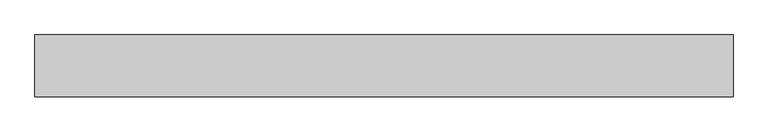
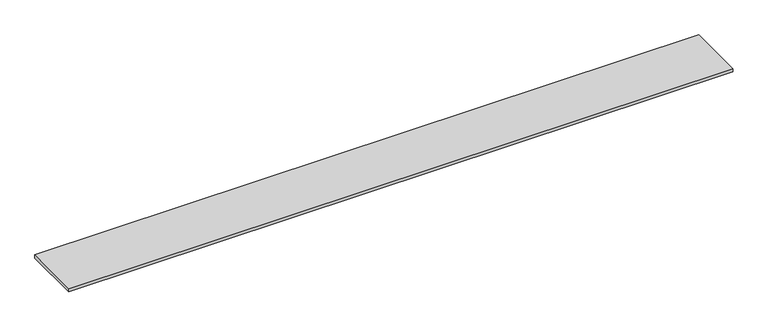
"""IFC4 building model written with IfcOpenShell, lengths in millimetres: proxy geometry, Generic Models 3:Generic Models 2:312240:Generic Models 2:312240 : Generic Models 3:Generic Models 2:312240:11 : Generic Models 3:Generic Models 2:312240:Generic Models 2:312240 : Generic Models 3:Generic Models 2:312240:300533."""

from ifc_helpers import new_model, si_unit, frame, origin, place, context, project, spatial, polyline, outline, extrude, source, transform, mapped, element, save


def generic_models_6350171e(model_context):
    return source(origin(), model_context, "Body", "SweptSolid", [
        extrude(outline(polyline([(592755.4242239, -578791.1413841), (592755.4242239, -579007.0413841), (590317.0242239, -579007.0413841), (590317.0242239, -578791.1413841), (592755.4242239, -578791.1413841)])), frame((0.0, 0.0, 1180.0460545), z_axis=(0.0, 0.0, 1.0), x_axis=(1.0, 0.0, 0.0)), (0.0, 0.0, 1.0), 12.364883),
    ])


if __name__ == "__main__":
    model = new_model("IFC4")
    model_context = context("Model", 3, world=origin())
    ifc_project = project(units=[si_unit("LENGTHUNIT", "METRE", prefix="MILLI")], contexts=[model_context])
    site = spatial("IfcSite", under=ifc_project)
    building = spatial("IfcBuilding", under=site)
    placement = place(None, origin())
    generic_models_shape = generic_models_6350171e(model_context)
    element("IfcBuildingElementProxy", 1, Name="Generic Models 3:Generic Models 2:312240:Generic Models 2:312240 : Generic Models 3:Generic Models 2:312240:11 : Generic Models 3:Generic Models 2:312240:Generic Models 2:312240 : Generic Models 3:Generic Models 2:312240:300533", ObjectType="Generic Models 3:Generic Models 2:312240:Generic Models 2:312240 : Generic Models 3:Generic Models 2:312240:11 : Generic Models 3:Generic Models 2:312240:Generic Models 2:312240 : Generic Models 3:Generic Models 2:312240:300533", at=placement, inside=building, context=model_context, shape_type="MappedRepresentation", body=[
        mapped(generic_models_shape, transform((0.0, 0.0, 0.0), x_axis=(1.0, 0.0, 0.0), y_axis=(0.0, 1.0, 0.0), z_axis=(0.0, 0.0, 1.0))),
    ])
    save(model, "model.ifc")

# Revit data of these elements
# Type "Generic Models 3:Generic Models 2:312240:Generic Models 2:312240 : Generic Models 3:Generic Models 2:312240:11 : Generic Models 3:Generic Models 2:312240:Generic Models 2:312240 : Generic Models 3:Generic Models 2:312240:300533"
#   NameOverride = "Generic Models 3:Generic Models 2:312240:Generic Models 2:312240 : Generic Models 3:Generic Models 2:312240:300533"
#   ObjectTypeOverride = "Generic Models 2:312240 : Generic Models 3:Generic Models 2:312240"
#   Reference = "Generic Models 2"
#   Tag = "300533"
# Element 1 (IfcBuildingElementProxy, "Generic Models 3:Generic Models 2:312240:Generic Models 2:312240 : Generic Models 3:Generic Models 2:312240:11 : Generic Models 3:Generic Models 2:312240:Generic Models 2:312240 : Generic Models 3:Generic Models 2:312240:300533")
#   Materials on its faces: "SOLID SURFACE MATERIAL (WITH HARD SEAMS, UNLESS OTHERWISE NOTED)"
# Materials
#   "SOLID SURFACE MATERIAL (WITH HARD SEAMS, UNLESS OTHERWISE NOTED)": class "Generic", colour RGB 242 242 242, transparency 0, Cost = 0
